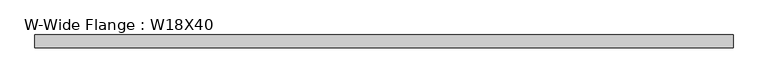
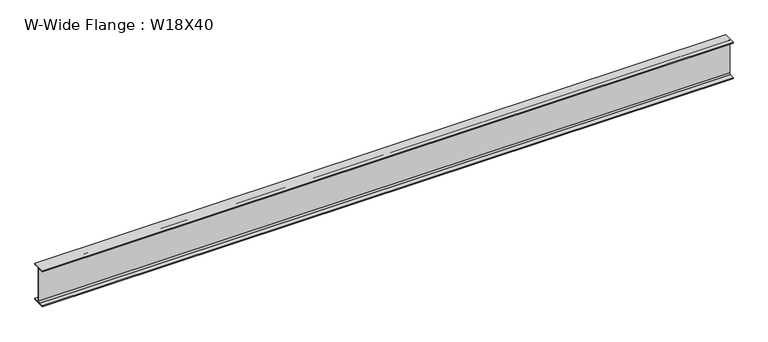
"""IFC4 building model written with IfcOpenShell, lengths in millimetres: beam geometry, W-Wide Flange : W18X40."""

from ifc_helpers import new_model, si_unit, point, frame, frame_2d, origin, place, context, project, spatial, polyline, circle_curve, trimmed, segment, composite_curve, outline, extrude, source, transform, mapped, element, save


def w_wide_flange_w18x40_b416f5d8(model_context):
    return source(origin(), model_context, "Body", "SweptSolid", [
        extrude(outline(composite_curve([segment(polyline([(76.454, -213.995), (76.454, -227.33), (-76.454, -227.33), (-76.454, -213.995), (-20.828, -213.995)]), True, "CONTINUOUS"), segment(trimmed(circle_curve(frame_2d((-20.828, -197.1675)), 16.8275), [point((-20.828, -213.995))], [point((-4.0005, -197.1675))], True, "CARTESIAN"), True, "CONTINUOUS"), segment(polyline([(-4.0005, -197.1675), (-4.0005, 197.1675)]), True, "CONTINUOUS"), segment(trimmed(circle_curve(frame_2d((-20.828, 197.1675)), 16.8275), [point((-4.0005, 197.1675))], [point((-20.828, 213.995))], True, "CARTESIAN"), True, "CONTINUOUS"), segment(polyline([(-20.828, 213.995), (-76.454, 213.995), (-76.454, 227.33), (76.454, 227.33), (76.454, 213.995), (20.828, 213.995)]), True, "CONTINUOUS"), segment(trimmed(circle_curve(frame_2d((20.828, 197.1675)), 16.8275), [point((20.828, 213.995))], [point((4.0005, 197.1675))], True, "CARTESIAN"), True, "CONTINUOUS"), segment(polyline([(4.0005, 197.1675), (4.0005, -197.1675)]), True, "CONTINUOUS"), segment(trimmed(circle_curve(frame_2d((20.828, -197.1675)), 16.8275), [point((4.0005, -197.1675))], [point((20.828, -213.995))], True, "CARTESIAN"), True, "CONTINUOUS"), segment(polyline([(20.828, -213.995), (76.454, -213.995)]), True, "CONTINUOUS")], self_intersect=False)), frame((-4095.75, 0.0, 0.0), z_axis=(1.0, 0.0, 0.0), x_axis=(0.0, 1.0, 0.0)), (0.0, 0.0, 1.0), 8191.5),
    ])


if __name__ == "__main__":
    model = new_model("IFC4")
    model_context = context("Model", 3, world=origin())
    ifc_project = project(units=[si_unit("LENGTHUNIT", "METRE", prefix="MILLI")], contexts=[model_context])
    site = spatial("IfcSite", under=ifc_project)
    building = spatial("IfcBuilding", under=site)
    placement = place(None, origin())
    w_wide_flange_w18x40_shape = w_wide_flange_w18x40_b416f5d8(model_context)
    element("IfcBeam", 1, ObjectType="W-Wide Flange : W18X40", at=placement, inside=building, context=model_context, shape_type="MappedRepresentation", body=[
        mapped(w_wide_flange_w18x40_shape, transform((0.0, 0.0, 0.0), x_axis=(1.0, 0.0, 0.0), y_axis=(0.0, 1.0, 0.0), z_axis=(0.0, 0.0, 1.0))),
    ])
    save(model, "model.ifc")

# Revit data of these elements
# Type "W-Wide Flange : W18X40"
#   Assembly Code = "B10"
#   W = 40
#   Length [instance default] = 5' - 0"
#   bf = 0' - 6.02"
#   d = 1' - 5.9"
#   k = 0' - 1 3/16"
#   k2 = 0' - 0.6625"
#   tf = 0' - 0.525"
#   tw = 0' - 0.315"
#   A = 0.0819444 SF
#   Structural Material [instance default] = Steel ASTM A992
# Element 1 (IfcBeam, "W-Wide Flange : W18X40")
#   Materials on its faces: "Steel ASTM A992"
# Materials
#   "Steel ASTM A992": class "Metal", colour RGB 199 199 199, transparency 0, Description = "Structural steel 50ksi", Cost = 0
